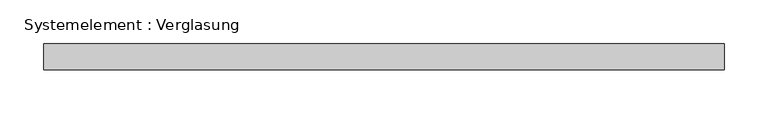
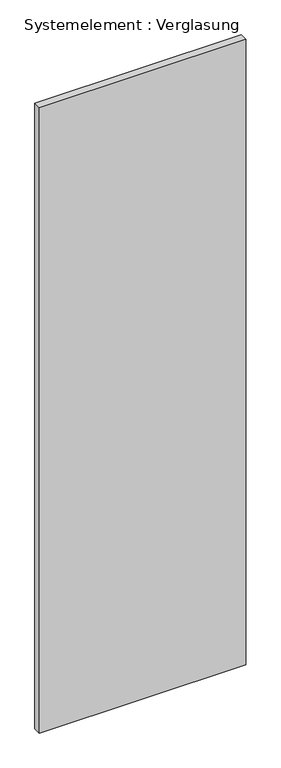
"""IFC4 building model written with IfcOpenShell, lengths in millimetres: plate geometry, Systemelement : Verglasung."""

from ifc_helpers import new_model, si_unit, origin, origin_with_axes, place, context, project, spatial, polyline, outline, extrude, source, transform, mapped, element, save


def systemelement_verglasung_11790072(model_context):
    return source(origin(), model_context, "Body", "SweptSolid", [
        extrude(outline(polyline([(390.3580711, -15.0), (-390.3580711, -15.0), (-390.3580711, 15.0), (390.3580711, 15.0), (390.3580711, -15.0)])), origin_with_axes(), (0.0, 0.0, 1.0), 2500.0),
    ])


if __name__ == "__main__":
    model = new_model("IFC4")
    model_context = context("Model", 3, world=origin())
    ifc_project = project(units=[si_unit("LENGTHUNIT", "METRE", prefix="MILLI")], contexts=[model_context])
    site = spatial("IfcSite", under=ifc_project)
    building = spatial("IfcBuilding", under=site)
    placement = place(None, origin())
    systemelement_verglasung_shape = systemelement_verglasung_11790072(model_context)
    element("IfcPlate", 1, ObjectType="Systemelement : Verglasung", at=placement, inside=building, context=model_context, shape_type="MappedRepresentation", body=[
        mapped(systemelement_verglasung_shape, transform((0.0, 0.0, 0.0), x_axis=(1.0, 0.0, 0.0), y_axis=(0.0, 1.0, 0.0), z_axis=(0.0, 0.0, 1.0))),
    ])
    save(model, "model.ifc")

# Revit data of these elements
# Type "Systemelement : Verglasung"
#   Construction Type Id = "GSP4R"
#   Analytic Construction = "1/8 Zoll Pilkington-Verglasung einfach"
#   Visual Light Transmittance = 0.9
#   Solar Heat Gain Coefficient = 0.86
#   Heat Transfer Coefficient (U) = 6.7069 W/(m²·K)
# Element 1 (IfcPlate, "Systemelement : Verglasung")
#   Materials on its faces: "Glas"
# Materials
#   "Glas": class "Glas", colour RGB 0 0 255, transparency 0.75, Comments = "Render-Darstellung nicht aktualisiert ", Cost = 0
